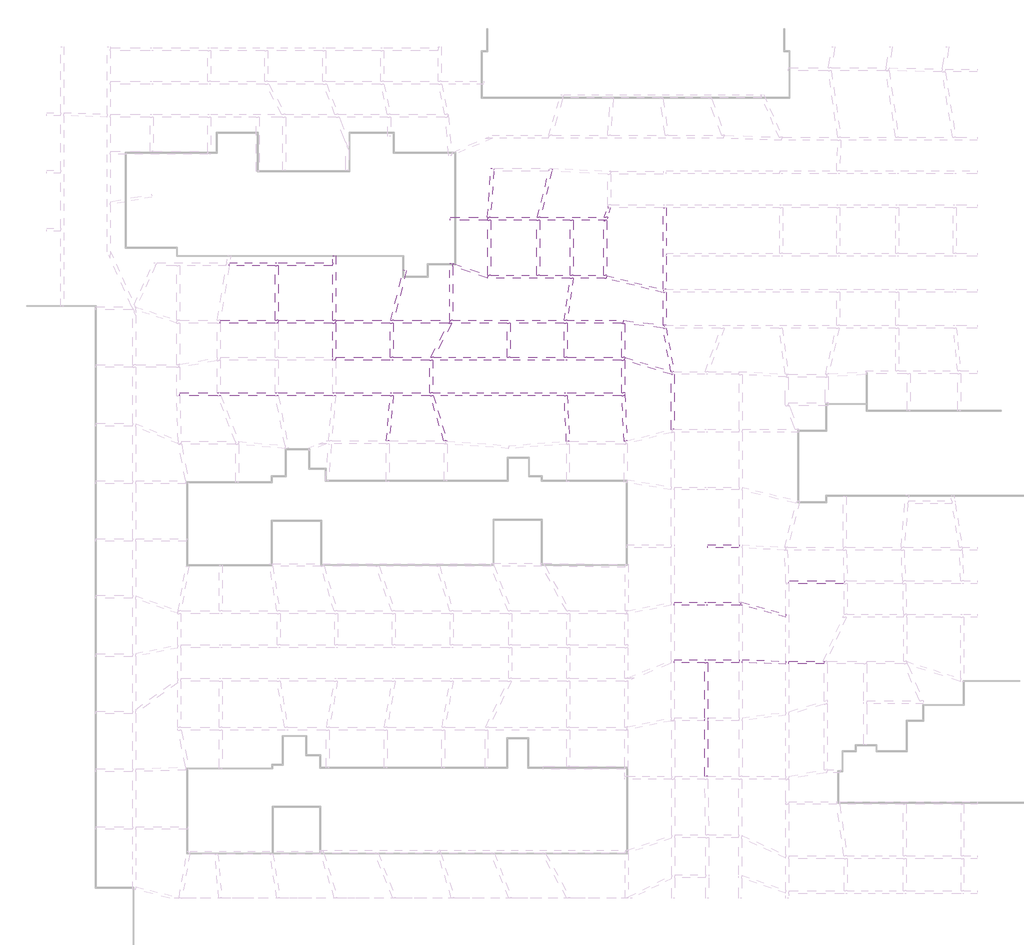
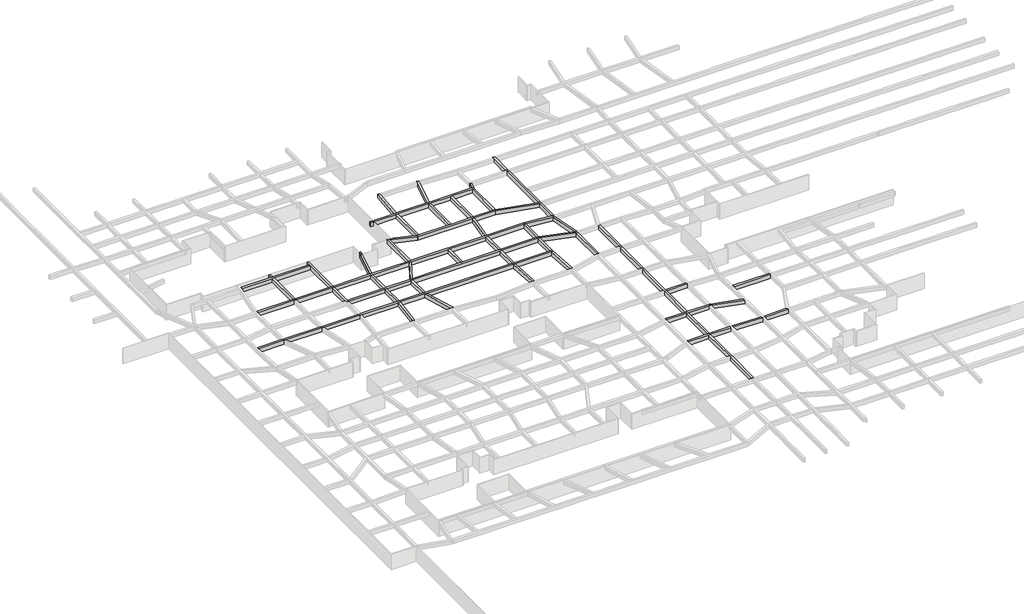
# One storey, part 16 of 45: 50 beams.
"""IFC4 building model written with IfcOpenShell, lengths in millimetres."""

from ifc_helpers import new_model, si_unit, frame, origin, place, context, project, spatial, polyline, outline, extrude, faceted_brep, element, save

model = new_model("IFC4")

# Units and contexts
model_context = context("Model", 3, world=origin())
ifc_project = project(units=[si_unit("LENGTHUNIT", "METRE", prefix="MILLI")], contexts=[model_context])

# Site, building, storey
site = spatial("IfcSite", under=ifc_project)
building = spatial("IfcBuilding", under=site)
storey = spatial("IfcBuildingStorey", under=building, Name="户型图", Elevation=0.0)

# Beams
placement = place(None, origin())
element("IfcBeam", 1, ObjectType="混凝土 - 矩形梁 : KL_beam", at=placement, inside=storey, context=model_context, shape_type="Brep", body=[
    faceted_brep([(-120998.6286131, -81886.7344834, 3300.0), (-120998.6286131, -81486.7344834, 3300.0), (-121398.6286131, -81486.7344834, 3300.0), (-128784.4586999, -81486.7344834, 3300.0), (-128818.6286131, -81486.7344834, 3300.0), (-128818.6286131, -81886.7344834, 3300.0), (-121398.6286131, -81886.7344834, 3300.0), (-120998.6286131, -81886.7344834, 2500.0), (-128818.6286131, -81886.7344834, 2500.0), (-121398.6286131, -81886.7344834, 2500.0), (-120998.6286131, -81486.7344834, 2500.0), (-128818.6286131, -81486.7344834, 2500.0), (-128784.4586999, -81486.7344834, 2500.0), (-121398.6286131, -81486.7344834, 2500.0)], [[[0, 1, 2, 3, 4, 5, 6]], [[7, 0, 6, 5, 8, 9]], [[10, 7, 9, 8, 11, 12, 13]], [[1, 10, 13, 12, 11, 4, 3, 2]], [[1, 0, 7, 10]], [[5, 4, 11, 8]]]),
])
element("IfcBeam", 2, ObjectType="混凝土 - 矩形梁 : KL_beam", at=placement, inside=storey, context=model_context, shape_type="Brep", body=[
    faceted_brep([(-113198.6286131, -81886.7344834, 3300.0), (-113198.6286131, -81486.7344834, 3300.0), (-113198.9292959, -81486.7344834, 3300.0), (-113598.9292959, -81486.7344834, 3300.0), (-120998.6286131, -81486.7344834, 3300.0), (-120998.6286131, -81886.7344834, 3300.0), (-113598.6286131, -81886.7344834, 3300.0), (-113198.6286131, -81886.7344834, 2500.0), (-120998.6286131, -81886.7344834, 2500.0), (-113598.6286131, -81886.7344834, 2500.0), (-113198.6286131, -81486.7344834, 2500.0), (-120998.6286131, -81486.7344834, 2500.0), (-113598.9292959, -81486.7344834, 2500.0), (-113198.9292959, -81486.7344834, 2500.0)], [[[0, 1, 2, 3, 4, 5, 6]], [[7, 0, 6, 5, 8, 9]], [[10, 7, 9, 8, 11, 12, 13]], [[1, 10, 13, 12, 11, 4, 3, 2]], [[5, 4, 11, 8]], [[1, 0, 7, 10]]]),
])
element("IfcBeam", 3, ObjectType="混凝土 - 矩形梁 : KL_beam", at=placement, inside=storey, context=model_context, shape_type="Brep", body=[
    faceted_brep([(-113598.6286131, -86886.7344834, 3300.0), (-113198.6286131, -86886.7344834, 3300.0), (-113198.6286131, -86486.7344834, 3300.0), (-113198.6286131, -81886.7344834, 3300.0), (-113598.6286131, -81886.7344834, 3300.0), (-113598.6286131, -86486.7344834, 3300.0), (-113598.6286131, -86886.7344834, 2500.0), (-113598.6286131, -81886.7344834, 2500.0), (-113598.6286131, -86486.7344834, 2500.0), (-113198.6286131, -86886.7344834, 2500.0), (-113198.6286131, -81886.7344834, 2500.0), (-113198.6286131, -86486.7344834, 2500.0)], [[[0, 1, 2, 3, 4, 5]], [[6, 0, 5, 4, 7, 8]], [[9, 6, 8, 7, 10, 11]], [[1, 9, 11, 10, 3, 2]], [[4, 3, 10, 7]], [[1, 0, 6, 9]]]),
])
element("IfcBeam", 4, ObjectType="混凝土 - 矩形梁 : KL_beam", at=placement, inside=storey, context=model_context, shape_type="SweptSolid", body=[
    extrude(outline(polyline([(-121398.6286131, -72759.2597696), (-120998.6286131, -72759.2597696), (-120998.6286131, -73686.7344834), (-121398.6286131, -73686.7344834), (-121398.6286131, -72759.2597696)])), frame((0.0, 0.0, 2500.0), z_axis=(0.0, 0.0, 1.0), x_axis=(1.0, 0.0, 0.0)), (0.0, 0.0, 1.0), 800.0),
    extrude(outline(polyline([(-120998.6286131, -81486.7344834), (-121398.6286131, -81486.7344834), (-121398.6286131, -74086.7344834), (-120998.6286131, -74086.7344834), (-120998.6286131, -81486.7344834)])), frame((0.0, 0.0, 2500.0), z_axis=(0.0, 0.0, 1.0), x_axis=(1.0, 0.0, 0.0)), (0.0, 0.0, 1.0), 800.0),
])
element("IfcBeam", 5, ObjectType="混凝土 - 矩形梁 : KL_beam", at=placement, inside=storey, context=model_context, shape_type="Brep", body=[
    faceted_brep([(-74128.0566076, -86886.7344834, 3300.0), (-74069.2006186, -86486.7344834, 3300.0), (-74098.3129002, -86486.7344834, 3300.0), (-74498.3129002, -86486.7344834, 3300.0), (-81898.3129002, -86486.7344834, 3300.0), (-82298.3129002, -86486.7344834, 3300.0), (-89598.3129002, -86486.7344834, 3300.0), (-89998.3129002, -86486.7344834, 3300.0), (-99914.2936835, -86486.7344834, 3300.0), (-100366.9162848, -86486.7344834, 3300.0), (-105392.6768411, -86486.7344834, 3300.0), (-105792.6768411, -86486.7344834, 3300.0), (-113198.6286131, -86486.7344834, 3300.0), (-113198.6286131, -86886.7344834, 3300.0), (-105792.6768411, -86886.7344834, 3300.0), (-105392.6768411, -86886.7344834, 3300.0), (-100446.5144021, -86886.7344834, 3300.0), (-100046.5144021, -86886.7344834, 3300.0), (-82298.3129002, -86886.7344834, 3300.0), (-81898.3129002, -86886.7344834, 3300.0), (-74498.3129002, -86886.7344834, 3300.0), (-74128.0566076, -86886.7344834, 2500.0), (-113198.6286131, -86886.7344834, 2500.0), (-105792.6768411, -86886.7344834, 2500.0), (-105392.6768411, -86886.7344834, 2500.0), (-100446.5144021, -86886.7344834, 2500.0), (-100046.5144021, -86886.7344834, 2500.0), (-82298.3129002, -86886.7344834, 2500.0), (-81898.3129002, -86886.7344834, 2500.0), (-74498.3129002, -86886.7344834, 2500.0), (-74069.2006186, -86486.7344834, 2500.0), (-113198.6286131, -86486.7344834, 2500.0), (-105792.6768411, -86486.7344834, 2500.0), (-105392.6768411, -86486.7344834, 2500.0), (-100366.9162848, -86486.7344834, 2500.0), (-99914.2936835, -86486.7344834, 2500.0), (-89998.3129002, -86486.7344834, 2500.0), (-89598.3129002, -86486.7344834, 2500.0), (-82298.3129002, -86486.7344834, 2500.0), (-81898.3129002, -86486.7344834, 2500.0), (-74498.3129002, -86486.7344834, 2500.0), (-74098.3129002, -86486.7344834, 2500.0)], [[[0, 1, 2, 3, 4, 5, 6, 7, 8, 9, 10, 11, 12, 13, 14, 15, 16, 17, 18, 19, 20]], [[21, 0, 20, 19, 18, 17, 16, 15, 14, 13, 22, 23, 24, 25, 26, 27, 28, 29]], [[30, 21, 29, 28, 27, 26, 25, 24, 23, 22, 31, 32, 33, 34, 35, 36, 37, 38, 39, 40, 41]], [[1, 30, 41, 40, 39, 38, 37, 36, 35, 34, 33, 32, 31, 12, 11, 10, 9, 8, 7, 6, 5, 4, 3, 2]], [[13, 12, 31, 22]], [[1, 0, 21, 30]]]),
])
element("IfcBeam", 6, ObjectType="混凝土 - 矩形梁 : KL_beam", at=placement, inside=storey, context=model_context, shape_type="Brep", body=[
    faceted_brep([(-74098.3129002, -91641.7669719, 3300.0), (-74098.3129002, -91436.9328993, 3300.0), (-74098.3129002, -91241.7669719, 3300.0), (-74498.3129002, -91241.7669719, 3300.0), (-81898.3129002, -91241.7669719, 3300.0), (-82298.3129002, -91241.7669719, 3300.0), (-100046.5144021, -91241.7669719, 3300.0), (-100446.5144021, -91241.7669719, 3300.0), (-105392.6768411, -91241.7669719, 3300.0), (-105792.6768411, -91241.7669719, 3300.0), (-113198.6286131, -91241.7669719, 3300.0), (-113598.6286131, -91241.7669719, 3300.0), (-120998.6286131, -91241.7669719, 3300.0), (-121398.6286131, -91241.7669719, 3300.0), (-128818.6286131, -91241.7669719, 3300.0), (-129218.6286131, -91241.7669719, 3300.0), (-134318.6286131, -91241.7669719, 3300.0), (-134318.6286131, -91641.7669719, 3300.0), (-134311.5225504, -91641.7669719, 3300.0), (-129156.0848049, -91641.7669719, 3300.0), (-128727.6268074, -91641.7669719, 3300.0), (-121363.4958903, -91641.7669719, 3300.0), (-120956.0092123, -91641.7669719, 3300.0), (-113616.8903133, -91641.7669719, 3300.0), (-113215.3623783, -91641.7669719, 3300.0), (-105810.9021134, -91641.7669719, 3300.0), (-105409.3741784, -91641.7669719, 3300.0), (-100395.5234862, -91641.7669719, 3300.0), (-99978.0743922, -91641.7669719, 3300.0), (-82288.8729227, -91641.7669719, 3300.0), (-81888.4052844, -91641.7669719, 3300.0), (-74488.8729227, -91641.7669719, 3300.0), (-74098.3129002, -91641.7669719, 2500.0), (-134318.6286131, -91641.7669719, 2500.0), (-134311.5225504, -91641.7669719, 2500.0), (-129156.0848049, -91641.7669719, 2500.0), (-128727.6268074, -91641.7669719, 2500.0), (-121363.4958903, -91641.7669719, 2500.0), (-120956.0092123, -91641.7669719, 2500.0), (-113616.8903133, -91641.7669719, 2500.0), (-113215.3623783, -91641.7669719, 2500.0), (-105810.9021134, -91641.7669719, 2500.0), (-105409.3741784, -91641.7669719, 2500.0), (-100395.5234862, -91641.7669719, 2500.0), (-99978.0743922, -91641.7669719, 2500.0), (-82288.8729227, -91641.7669719, 2500.0), (-81888.4052844, -91641.7669719, 2500.0), (-74488.8729227, -91641.7669719, 2500.0), (-74098.3129002, -91241.7669719, 2500.0), (-74098.3129002, -91436.9328993, 2500.0), (-134318.6286131, -91241.7669719, 2500.0), (-129218.6286131, -91241.7669719, 2500.0), (-128818.6286131, -91241.7669719, 2500.0), (-121398.6286131, -91241.7669719, 2500.0), (-120998.6286131, -91241.7669719, 2500.0), (-113598.6286131, -91241.7669719, 2500.0), (-113198.6286131, -91241.7669719, 2500.0), (-105792.6768411, -91241.7669719, 2500.0), (-105392.6768411, -91241.7669719, 2500.0), (-100446.5144021, -91241.7669719, 2500.0), (-100046.5144021, -91241.7669719, 2500.0), (-82298.3129002, -91241.7669719, 2500.0), (-81898.3129002, -91241.7669719, 2500.0), (-74498.3129002, -91241.7669719, 2500.0)], [[[0, 1, 2, 3, 4, 5, 6, 7, 8, 9, 10, 11, 12, 13, 14, 15, 16, 17, 18, 19, 20, 21, 22, 23, 24, 25, 26, 27, 28, 29, 30, 31]], [[32, 0, 31, 30, 29, 28, 27, 26, 25, 24, 23, 22, 21, 20, 19, 18, 17, 33, 34, 35, 36, 37, 38, 39, 40, 41, 42, 43, 44, 45, 46, 47]], [[48, 49, 32, 47, 46, 45, 44, 43, 42, 41, 40, 39, 38, 37, 36, 35, 34, 33, 50, 51, 52, 53, 54, 55, 56, 57, 58, 59, 60, 61, 62, 63]], [[2, 48, 63, 62, 61, 60, 59, 58, 57, 56, 55, 54, 53, 52, 51, 50, 16, 15, 14, 13, 12, 11, 10, 9, 8, 7, 6, 5, 4, 3]], [[17, 16, 50, 33]], [[2, 1, 0, 32, 49, 48]]]),
])
element("IfcBeam", 7, ObjectType="混凝土 - 矩形梁 : KL_beam", at=placement, inside=storey, context=model_context, shape_type="SweptSolid", body=[
    extrude(outline(polyline([(-105810.9021134, -91641.7669719), (-105409.3741784, -91641.7669719), (-105946.1060855, -97776.6407423), (-106347.6340205, -97776.6407423), (-105810.9021134, -91641.7669719)])), frame((0.0, 0.0, 2500.0), z_axis=(0.0, 0.0, 1.0), x_axis=(1.0, 0.0, 0.0)), (0.0, 0.0, 1.0), 800.0),
])
element("IfcBeam", 8, ObjectType="混凝土 - 矩形梁 : KL_beam", at=placement, inside=storey, context=model_context, shape_type="Brep", body=[
    faceted_brep([(-92598.5285941, -67552.5441851, 3300.0), (-92598.5285941, -67552.7981742, 3300.0), (-92598.5285941, -67952.5441851, 3300.0), (-92198.5285941, -67952.5441851, 3300.0), (-85971.6416274, -67952.5441851, 3300.0), (-85571.6416274, -67952.5441851, 3300.0), (-81471.6416274, -67952.5441851, 3300.0), (-81071.6416274, -67952.5441851, 3300.0), (-76547.2291492, -67952.5441851, 3300.0), (-76434.1522111, -67552.5441851, 3300.0), (-76849.828039, -67552.5441851, 3300.0), (-85515.5899744, -67552.5441851, 3300.0), (-85927.8354261, -67552.5441851, 3300.0), (-92270.5908787, -67552.5441851, 3300.0), (-92598.5285941, -67952.5441851, 2500.0), (-92198.5285941, -67952.5441851, 2500.0), (-85971.6416274, -67952.5441851, 2500.0), (-85571.6416274, -67952.5441851, 2500.0), (-81471.6416274, -67952.5441851, 2500.0), (-81071.6416274, -67952.5441851, 2500.0), (-76547.2291492, -67952.5441851, 2500.0), (-92598.5285941, -67552.7981742, 2500.0), (-92598.5285941, -67552.5441851, 2500.0), (-92270.5908787, -67552.5441851, 2500.0), (-85927.8354261, -67552.5441851, 2500.0), (-85515.5899744, -67552.5441851, 2500.0), (-76849.828039, -67552.5441851, 2500.0), (-76434.1522111, -67552.5441851, 2500.0)], [[[0, 1, 2, 3, 4, 5, 6, 7, 8, 9, 10, 11, 12, 13]], [[2, 14, 15, 16, 17, 18, 19, 20, 8, 7, 6, 5, 4, 3]], [[14, 21, 22, 23, 24, 25, 26, 27, 20, 19, 18, 17, 16, 15]], [[22, 0, 13, 12, 11, 10, 9, 27, 26, 25, 24, 23]], [[2, 1, 0, 22, 21, 14]], [[9, 8, 20, 27]]]),
])
element("IfcBeam", 9, ObjectType="混凝土 - 矩形梁 : KL_beam", at=placement, inside=storey, context=model_context, shape_type="Brep", body=[
    faceted_brep([(-92598.5285941, -75365.0521634, 3300.0), (-92598.5285941, -75765.0521634, 3300.0), (-81500.4649427, -75765.0521634, 3300.0), (-81096.8342659, -75765.0521634, 3300.0), (-76794.8911053, -75765.0521634, 3300.0), (-76570.1397921, -75765.0521634, 3300.0), (-76570.1397921, -75408.8435077, 3300.0), (-76570.1397921, -75365.0521634, 3300.0), (-76970.1397921, -75365.0521634, 3300.0), (-81071.6416274, -75365.0521634, 3300.0), (-81471.6416274, -75365.0521634, 3300.0), (-85571.6416274, -75365.0521634, 3300.0), (-85971.6416274, -75365.0521634, 3300.0), (-92198.5285941, -75365.0521634, 3300.0), (-92598.5285941, -75765.0521634, 2500.0), (-81500.4649427, -75765.0521634, 2500.0), (-81096.8342659, -75765.0521634, 2500.0), (-76794.8911053, -75765.0521634, 2500.0), (-76570.1397921, -75765.0521634, 2500.0), (-92598.5285941, -75365.0521634, 2500.0), (-92198.5285941, -75365.0521634, 2500.0), (-85971.6416274, -75365.0521634, 2500.0), (-85571.6416274, -75365.0521634, 2500.0), (-81471.6416274, -75365.0521634, 2500.0), (-81071.6416274, -75365.0521634, 2500.0), (-76970.1397921, -75365.0521634, 2500.0), (-76570.1397921, -75365.0521634, 2500.0), (-76570.1397921, -75408.8435077, 2500.0)], [[[0, 1, 2, 3, 4, 5, 6, 7, 8, 9, 10, 11, 12, 13]], [[1, 14, 15, 16, 17, 18, 5, 4, 3, 2]], [[14, 19, 20, 21, 22, 23, 24, 25, 26, 27, 18, 17, 16, 15]], [[19, 0, 13, 12, 11, 10, 9, 8, 7, 26, 25, 24, 23, 22, 21, 20]], [[1, 0, 19, 14]], [[7, 6, 5, 18, 27, 26]]]),
])
element("IfcBeam", 10, ObjectType="混凝土 - 矩形梁 : KL_beam", at=placement, inside=storey, context=model_context, shape_type="Brep", body=[
    faceted_brep([(-74310.2286213, -81886.7344834, 3300.0), (-74287.028605, -81486.7344834, 3300.0), (-81869.489585, -81486.7344834, 3300.0), (-82273.1202618, -81486.7344834, 3300.0), (-97398.6286131, -81486.7344834, 3300.0), (-97798.6286131, -81486.7344834, 3300.0), (-97798.6286131, -81886.7344834, 3300.0), (-97478.3770718, -81886.7344834, 3300.0), (-89998.3129002, -81886.7344834, 3300.0), (-89598.3129002, -81886.7344834, 3300.0), (-82298.3129002, -81886.7344834, 3300.0), (-81898.3129002, -81886.7344834, 3300.0), (-74498.3129002, -81886.7344834, 3300.0), (-74310.2286213, -81886.7344834, 2500.0), (-97798.6286131, -81886.7344834, 2500.0), (-97478.3770718, -81886.7344834, 2500.0), (-89998.3129002, -81886.7344834, 2500.0), (-89598.3129002, -81886.7344834, 2500.0), (-82298.3129002, -81886.7344834, 2500.0), (-81898.3129002, -81886.7344834, 2500.0), (-74498.3129002, -81886.7344834, 2500.0), (-74287.028605, -81486.7344834, 2500.0), (-97798.6286131, -81486.7344834, 2500.0), (-97398.6286131, -81486.7344834, 2500.0), (-82273.1202618, -81486.7344834, 2500.0), (-81869.489585, -81486.7344834, 2500.0)], [[[0, 1, 2, 3, 4, 5, 6, 7, 8, 9, 10, 11, 12]], [[13, 0, 12, 11, 10, 9, 8, 7, 6, 14, 15, 16, 17, 18, 19, 20]], [[21, 13, 20, 19, 18, 17, 16, 15, 14, 22, 23, 24, 25]], [[1, 21, 25, 24, 23, 22, 5, 4, 3, 2]], [[1, 0, 13, 21]], [[6, 5, 22, 14]]]),
])
element("IfcBeam", 11, ObjectType="混凝土 - 矩形梁 : KL_beam", at=placement, inside=storey, context=model_context, shape_type="SweptSolid", body=[
    extrude(outline(polyline([(-85971.6416274, -67952.5441851), (-85571.6416274, -67952.5441851), (-85571.6416274, -75365.0521634), (-85971.6416274, -75365.0521634), (-85971.6416274, -67952.5441851)])), frame((0.0, 0.0, 2500.0), z_axis=(0.0, 0.0, 1.0), x_axis=(1.0, 0.0, 0.0)), (0.0, 0.0, 1.0), 800.0),
])
element("IfcBeam", 12, ObjectType="混凝土 - 矩形梁 : KL_beam", at=placement, inside=storey, context=model_context, shape_type="SweptSolid", body=[
    extrude(outline(polyline([(-81471.6416274, -67952.5441851), (-81071.6416274, -67952.5441851), (-81071.6416274, -75365.0521634), (-81471.6416274, -75365.0521634), (-81471.6416274, -67952.5441851)])), frame((0.0, 0.0, 2500.0), z_axis=(0.0, 0.0, 1.0), x_axis=(1.0, 0.0, 0.0)), (0.0, 0.0, 1.0), 800.0),
])
element("IfcBeam", 13, ObjectType="混凝土 - 矩形梁 : KL_beam", at=placement, inside=storey, context=model_context, shape_type="Brep", body=[
    faceted_brep([(-92198.5285941, -67952.5441851, 3300.0), (-92598.5285941, -67952.5441851, 3300.0), (-92598.5285941, -67952.7981742, 3300.0), (-92598.5285941, -75353.8354852, 3300.0), (-92598.5285941, -75365.0521634, 3300.0), (-92198.5285941, -75365.0521634, 3300.0), (-92598.5285941, -67952.5441851, 2500.0), (-92598.5285941, -67952.7981742, 2500.0), (-92598.5285941, -75353.8354852, 2500.0), (-92598.5285941, -75365.0521634, 2500.0), (-92198.5285941, -67952.5441851, 2500.0), (-92198.5285941, -75365.0521634, 2500.0)], [[[0, 1, 2, 3, 4, 5]], [[1, 6, 7, 8, 9, 4, 3, 2]], [[6, 10, 11, 9, 8, 7]], [[10, 0, 5, 11]], [[1, 0, 10, 6]], [[5, 4, 9, 11]]]),
])
element("IfcBeam", 14, ObjectType="混凝土 - 矩形梁 : KL_beam", at=placement, inside=storey, context=model_context, shape_type="Brep", body=[
    faceted_brep([(-68721.961123, -82134.4617231, 3300.0), (-68900.6999587, -82113.6580198, 3300.0), (-74287.028605, -81486.7344834, 3300.0), (-74310.2286213, -81886.7344834, 3300.0), (-74098.3129002, -81911.3996982, 3300.0), (-68904.9700465, -82515.8613049, 3300.0), (-68745.1611393, -82534.4617231, 3300.0), (-74310.2286213, -81886.7344834, 2500.0), (-74098.3129002, -81911.3996982, 2500.0), (-68904.9700465, -82515.8613049, 2500.0), (-68745.1611393, -82534.4617231, 2500.0), (-74287.028605, -81486.7344834, 2500.0), (-68900.6999587, -82113.6580198, 2500.0), (-68721.961123, -82134.4617231, 2500.0)], [[[0, 1, 2, 3, 4, 5, 6]], [[6, 5, 4, 3, 7, 8, 9, 10]], [[10, 9, 8, 7, 11, 12, 13]], [[2, 1, 0, 13, 12, 11]], [[2, 11, 7, 3]], [[0, 6, 10, 13]]]),
])
element("IfcBeam", 15, ObjectType="混凝土 - 矩形梁 : KL_beam", at=placement, inside=storey, context=model_context, shape_type="Brep", body=[
    faceted_brep([(-67740.4118212, -88390.3844516, 3300.0), (-67876.3425814, -88349.4975464, 3300.0), (-74069.2006186, -86486.7344834, 3300.0), (-74128.0566076, -86886.7344834, 3300.0), (-74098.3129002, -86895.681157, 3300.0), (-67830.7823984, -88780.9051109, 3300.0), (-67799.2678102, -88790.3844516, 3300.0), (-74128.0566076, -86886.7344834, 2500.0), (-74098.3129002, -86895.681157, 2500.0), (-67830.7823984, -88780.9051109, 2500.0), (-67799.2678102, -88790.3844516, 2500.0), (-74069.2006186, -86486.7344834, 2500.0), (-67876.3425814, -88349.4975464, 2500.0), (-67740.4118212, -88390.3844516, 2500.0)], [[[0, 1, 2, 3, 4, 5, 6]], [[6, 5, 4, 3, 7, 8, 9, 10]], [[10, 9, 8, 7, 11, 12, 13]], [[2, 1, 0, 13, 12, 11]], [[2, 11, 7, 3]], [[0, 6, 10, 13]]]),
])
element("IfcBeam", 16, ObjectType="混凝土 - 矩形梁 : KL_beam", at=placement, inside=storey, context=model_context, shape_type="SweptSolid", body=[
    extrude(outline(polyline([(-74310.2286213, -81886.7344834), (-74098.3129002, -81911.3996982), (-74098.3129002, -86486.7344834), (-74498.3129002, -86486.7344834), (-74498.3129002, -81886.7344834), (-74310.2286213, -81886.7344834)])), frame((0.0, 0.0, 2500.0), z_axis=(0.0, 0.0, 1.0), x_axis=(1.0, 0.0, 0.0)), (0.0, 0.0, 1.0), 800.0),
])
element("IfcBeam", 17, ObjectType="混凝土 - 矩形梁 : KL_beam", at=placement, inside=storey, context=model_context, shape_type="SweptSolid", body=[
    extrude(outline(polyline([(-74098.3129002, -91241.7669719), (-74498.3129002, -91241.7669719), (-74498.3129002, -86886.7344834), (-74128.0566076, -86886.7344834), (-74098.3129002, -86895.681157), (-74098.3129002, -91241.7669719)])), frame((0.0, 0.0, 2500.0), z_axis=(0.0, 0.0, 1.0), x_axis=(1.0, 0.0, 0.0)), (0.0, 0.0, 1.0), 800.0),
])
element("IfcBeam", 18, ObjectType="混凝土 - 矩形梁 : KL_beam", at=placement, inside=storey, context=model_context, shape_type="SweptSolid", body=[
    extrude(outline(polyline([(-74488.8729227, -91641.7669719), (-74098.3129002, -91641.7669719), (-74098.3129002, -91436.9328993), (-73792.8353015, -97752.5007811), (-74005.7852131, -97806.5978244), (-74190.6863209, -97806.5978244), (-74488.8729227, -91641.7669719)])), frame((0.0, 0.0, 2500.0), z_axis=(0.0, 0.0, 1.0), x_axis=(1.0, 0.0, 0.0)), (0.0, 0.0, 1.0), 800.0),
])
element("IfcBeam", 19, ObjectType="混凝土 - 矩形梁 : KL_beam", at=placement, inside=storey, context=model_context, shape_type="SweptSolid", body=[
    extrude(outline(polyline([(-81590.2186825, -97806.5978244), (-81990.6863209, -97806.5978244), (-82288.8729227, -91641.7669719), (-81888.4052844, -91641.7669719), (-81590.2186825, -97806.5978244)])), frame((0.0, 0.0, 2500.0), z_axis=(0.0, 0.0, 1.0), x_axis=(1.0, 0.0, 0.0)), (0.0, 0.0, 1.0), 800.0),
])
element("IfcBeam", 20, ObjectType="混凝土 - 矩形梁 : KL_beam", at=placement, inside=storey, context=model_context, shape_type="SweptSolid", body=[
    extrude(outline(polyline([(-81898.3129002, -91241.7669719), (-82298.3129002, -91241.7669719), (-82298.3129002, -86886.7344834), (-81898.3129002, -86886.7344834), (-81898.3129002, -91241.7669719)])), frame((0.0, 0.0, 2500.0), z_axis=(0.0, 0.0, 1.0), x_axis=(1.0, 0.0, 0.0)), (0.0, 0.0, 1.0), 800.0),
    extrude(outline(polyline([(-82298.3129002, -81886.7344834), (-81898.3129002, -81886.7344834), (-81898.3129002, -86486.7344834), (-82298.3129002, -86486.7344834), (-82298.3129002, -81886.7344834)])), frame((0.0, 0.0, 2500.0), z_axis=(0.0, 0.0, 1.0), x_axis=(1.0, 0.0, 0.0)), (0.0, 0.0, 1.0), 800.0),
])
element("IfcBeam", 21, ObjectType="混凝土 - 矩形梁 : KL_beam", at=placement, inside=storey, context=model_context, shape_type="SweptSolid", body=[
    extrude(outline(polyline([(-81500.4649427, -75765.0521634), (-81096.8342659, -75765.0521634), (-81869.489585, -81486.7344834), (-82273.1202618, -81486.7344834), (-81500.4649427, -75765.0521634)])), frame((0.0, 0.0, 2500.0), z_axis=(0.0, 0.0, 1.0), x_axis=(1.0, 0.0, 0.0)), (0.0, 0.0, 1.0), 800.0),
])
element("IfcBeam", 22, ObjectType="混凝土 - 矩形梁 : KL_beam", at=placement, inside=storey, context=model_context, shape_type="SweptSolid", body=[
    extrude(outline(polyline([(-89598.3129002, -86486.7344834), (-89998.3129002, -86486.7344834), (-89998.3129002, -81886.7344834), (-89598.3129002, -81886.7344834), (-89598.3129002, -86486.7344834)])), frame((0.0, 0.0, 2500.0), z_axis=(0.0, 0.0, 1.0), x_axis=(1.0, 0.0, 0.0)), (0.0, 0.0, 1.0), 800.0),
])
element("IfcBeam", 23, ObjectType="混凝土 - 矩形梁 : KL_beam", at=placement, inside=storey, context=model_context, shape_type="SweptSolid", body=[
    extrude(outline(polyline([(-68904.9700465, -82515.8613049), (-68745.1611393, -82534.4617231), (-68495.5196461, -82534.4617231), (-67462.9624722, -88390.3844516), (-67740.4118212, -88390.3844516), (-67876.3425814, -88349.4975464), (-68904.9700465, -82515.8613049)])), frame((0.0, 0.0, 2500.0), z_axis=(0.0, 0.0, 1.0), x_axis=(1.0, 0.0, 0.0)), (0.0, 0.0, 1.0), 800.0),
])
element("IfcBeam", 24, ObjectType="混凝土 - 矩形梁 : KL_beam", at=placement, inside=storey, context=model_context, shape_type="Brep", body=[
    faceted_brep([(-67725.9320986, -96211.286122, 3300.0), (-67430.7823984, -96211.286122, 3300.0), (-67430.7823984, -88790.3844516, 3300.0), (-67798.6023246, -88790.3844516, 3300.0), (-67799.2678102, -88790.3844516, 3300.0), (-67830.7823984, -88780.9051109, 3300.0), (-67830.7823984, -96237.9219218, 3300.0), (-67830.7823984, -88780.9051109, 2500.0), (-67830.7823984, -96237.9219218, 2500.0), (-67430.7823984, -96211.286122, 2500.0), (-67725.9320986, -96211.286122, 2500.0), (-67799.2678102, -88790.3844516, 2500.0), (-67798.6023246, -88790.3844516, 2500.0), (-67430.7823984, -88790.3844516, 2500.0)], [[[0, 1, 2, 3, 4, 5, 6]], [[5, 7, 8, 6]], [[9, 10, 8, 7, 11, 12, 13]], [[1, 9, 13, 2]], [[1, 0, 10, 9]], [[2, 13, 12, 11, 4, 3]], [[5, 4, 11, 7]], [[0, 6, 8, 10]]]),
])
element("IfcBeam", 25, ObjectType="混凝土 - 矩形梁 : KL_beam", at=placement, inside=storey, context=model_context, shape_type="Brep", body=[
    faceted_brep([(-58457.1128979, -119970.4077047, 3300.0), (-58404.4518989, -119570.4077047, 3300.0), (-58630.7823984, -119570.4077047, 3300.0), (-62877.6696197, -119570.4077047, 3300.0), (-63277.6696197, -119570.4077047, 3300.0), (-67430.7823984, -119570.4077047, 3300.0), (-67430.7823984, -119970.4077047, 3300.0), (-63277.6696197, -119970.4077047, 3300.0), (-62877.6696197, -119970.4077047, 3300.0), (-58630.7823984, -119970.4077047, 3300.0), (-58457.1128979, -119970.4077047, 2500.0), (-67430.7823984, -119970.4077047, 2500.0), (-63277.6696197, -119970.4077047, 2500.0), (-62877.6696197, -119970.4077047, 2500.0), (-58630.7823984, -119970.4077047, 2500.0), (-58404.4518989, -119570.4077047, 2500.0), (-67430.7823984, -119570.4077047, 2500.0), (-63277.6696197, -119570.4077047, 2500.0), (-62877.6696197, -119570.4077047, 2500.0), (-58630.7823984, -119570.4077047, 2500.0)], [[[0, 1, 2, 3, 4, 5, 6, 7, 8, 9]], [[10, 0, 9, 8, 7, 6, 11, 12, 13, 14]], [[15, 10, 14, 13, 12, 11, 16, 17, 18, 19]], [[1, 15, 19, 18, 17, 16, 5, 4, 3, 2]], [[6, 5, 16, 11]], [[1, 0, 10, 15]]]),
])
element("IfcBeam", 26, ObjectType="混凝土 - 矩形梁 : KL_beam", at=placement, inside=storey, context=model_context, shape_type="Brep", body=[
    faceted_brep([(-67430.7823984, -127365.3480623, 3300.0), (-67430.7823984, -127765.3480623, 3300.0), (-63277.6696197, -127765.3480623, 3300.0), (-62877.6696197, -127765.3480623, 3300.0), (-58630.7823984, -127765.3480623, 3300.0), (-58630.7823984, -127365.3480623, 3300.0), (-62877.6696197, -127365.3480623, 3300.0), (-63277.6696197, -127365.3480623, 3300.0), (-67430.7823984, -127765.3480623, 2500.0), (-63277.6696197, -127765.3480623, 2500.0), (-62877.6696197, -127765.3480623, 2500.0), (-58630.7823984, -127765.3480623, 2500.0), (-67430.7823984, -127365.3480623, 2500.0), (-63277.6696197, -127365.3480623, 2500.0), (-62877.6696197, -127365.3480623, 2500.0), (-58630.7823984, -127365.3480623, 2500.0)], [[[0, 1, 2, 3, 4, 5, 6, 7]], [[1, 8, 9, 10, 11, 4, 3, 2]], [[8, 12, 13, 14, 15, 11, 10, 9]], [[12, 0, 7, 6, 5, 15, 14, 13]], [[1, 0, 12, 8]], [[5, 4, 11, 15]]]),
])
element("IfcBeam", 27, ObjectType="混凝土 - 矩形梁 : KL_beam", at=placement, inside=storey, context=model_context, shape_type="SweptSolid", body=[
    extrude(outline(polyline([(-58230.7823984, -127768.9840855), (-58230.7823984, -127368.7402678), (-52297.3620817, -127575.9398709), (-52297.3620817, -127976.1836887), (-58230.7823984, -127768.9840855)])), frame((0.0, 0.0, 2500.0), z_axis=(0.0, 0.0, 1.0), x_axis=(1.0, 0.0, 0.0)), (0.0, 0.0, 1.0), 800.0),
])
element("IfcBeam", 28, ObjectType="混凝土 - 矩形梁 : KL_beam", at=placement, inside=storey, context=model_context, shape_type="Brep", body=[
    faceted_brep([(-58404.4518989, -119570.4077047, 3300.0), (-58457.1128979, -119970.4077047, 3300.0), (-58230.7823984, -120031.0527792, 3300.0), (-52297.3620817, -121620.9079614, 3300.0), (-52297.3620817, -121206.7974893, 3300.0), (-58230.7823984, -119616.9423071, 3300.0), (-58457.1128979, -119970.4077047, 2500.0), (-58230.7823984, -120031.0527792, 2500.0), (-52297.3620817, -121620.9079614, 2500.0), (-58404.4518989, -119570.4077047, 2500.0), (-58230.7823984, -119616.9423071, 2500.0), (-52297.3620817, -121206.7974893, 2500.0)], [[[0, 1, 2, 3, 4, 5]], [[1, 6, 7, 8, 3, 2]], [[6, 9, 10, 11, 8, 7]], [[9, 0, 5, 4, 11, 10]], [[0, 9, 6, 1]], [[4, 3, 8, 11]]]),
])
element("IfcBeam", 29, ObjectType="混凝土 - 矩形梁 : KL_beam", at=placement, inside=storey, context=model_context, shape_type="Brep", body=[
    faceted_brep([(-47087.6738698, -127942.8806028, 3300.0), (-47087.6738698, -127542.8806028, 3300.0), (-47222.4961059, -127542.8806028, 3300.0), (-51897.3620817, -127542.8806028, 3300.0), (-51897.3620817, -127942.8806028, 3300.0), (-47087.6738698, -127542.8806028, 2500.0), (-47222.4961059, -127542.8806028, 2500.0), (-51897.3620817, -127542.8806028, 2500.0), (-47087.6738698, -127942.8806028, 2500.0), (-51897.3620817, -127942.8806028, 2500.0)], [[[0, 1, 2, 3, 4]], [[1, 5, 6, 7, 3, 2]], [[5, 8, 9, 7, 6]], [[8, 0, 4, 9]], [[1, 0, 8, 5]], [[3, 7, 9, 4]]]),
])
element("IfcBeam", 30, ObjectType="混凝土 - 矩形梁 : KL_beam", at=placement, inside=storey, context=model_context, shape_type="Brep", body=[
    faceted_brep([(-51907.4445387, -116668.4603553, 3300.0), (-51886.481427, -117068.4603553, 3300.0), (-44392.4702803, -117068.4603553, 3300.0), (-44385.6244664, -117068.4603553, 3300.0), (-44399.5927742, -116668.4603553, 3300.0), (-51886.481427, -117068.4603553, 2500.0), (-44392.4702803, -117068.4603553, 2500.0), (-44385.6244664, -117068.4603553, 2500.0), (-51907.4445387, -116668.4603553, 2500.0), (-44399.5927742, -116668.4603553, 2500.0)], [[[0, 1, 2, 3, 4]], [[1, 5, 6, 7, 3, 2]], [[5, 8, 9, 7, 6]], [[8, 0, 4, 9]], [[1, 0, 8, 5]], [[4, 3, 7, 9]]]),
])
element("IfcBeam", 31, ObjectType="混凝土 - 矩形梁 : KL_beam", at=placement, inside=storey, context=model_context, shape_type="SweptSolid", body=[
    extrude(outline(polyline([(-58630.7823984, -111828.4346923), (-58630.7823984, -112228.4346923), (-62877.6696197, -112228.4346923), (-62877.6696197, -111828.4346923), (-58630.7823984, -111828.4346923)])), frame((0.0, 0.0, 2500.0), z_axis=(0.0, 0.0, 1.0), x_axis=(1.0, 0.0, 0.0)), (0.0, 0.0, 1.0), 800.0),
])
element("IfcBeam", 32, ObjectType="混凝土 - 矩形梁 : KL_beam", at=placement, inside=storey, context=model_context, shape_type="SweptSolid", body=[
    extrude(outline(polyline([(-105392.6768411, -91241.7669719), (-105792.6768411, -91241.7669719), (-105792.6768411, -86886.7344834), (-105392.6768411, -86886.7344834), (-105392.6768411, -91241.7669719)])), frame((0.0, 0.0, 2500.0), z_axis=(0.0, 0.0, 1.0), x_axis=(1.0, 0.0, 0.0)), (0.0, 0.0, 1.0), 800.0),
    extrude(outline(polyline([(-105392.6768411, -86486.7344834), (-105792.6768411, -86486.7344834), (-105792.6768411, -81886.7344834), (-105392.6768411, -81886.7344834), (-105392.6768411, -86486.7344834)])), frame((0.0, 0.0, 2500.0), z_axis=(0.0, 0.0, 1.0), x_axis=(1.0, 0.0, 0.0)), (0.0, 0.0, 1.0), 800.0),
])
element("IfcBeam", 33, ObjectType="混凝土 - 矩形梁 : KL_beam", at=placement, inside=storey, context=model_context, shape_type="SweptSolid", body=[
    extrude(outline(polyline([(-104045.0172739, -74652.7141451), (-103656.8989834, -74749.4829033), (-105336.6844645, -81486.7344834), (-105748.9299162, -81486.7344834), (-104045.0172739, -74652.7141451)])), frame((0.0, 0.0, 2500.0), z_axis=(0.0, 0.0, 1.0), x_axis=(1.0, 0.0, 0.0)), (0.0, 0.0, 1.0), 800.0),
])
element("IfcBeam", 34, ObjectType="混凝土 - 矩形梁 : KL_beam", at=placement, inside=storey, context=model_context, shape_type="Brep", body=[
    faceted_brep([(-113198.6286131, -81486.7344834, 3300.0), (-113198.6286131, -81886.7344834, 3300.0), (-105792.6768411, -81886.7344834, 3300.0), (-105392.6768411, -81886.7344834, 3300.0), (-97930.999673, -81886.7344834, 3300.0), (-97798.6286131, -81886.7344834, 3300.0), (-97798.6286131, -81486.7344834, 3300.0), (-105336.6844645, -81486.7344834, 3300.0), (-105748.9299162, -81486.7344834, 3300.0), (-113198.6286131, -81486.7344834, 2500.0), (-97798.6286131, -81486.7344834, 2500.0), (-105336.6844645, -81486.7344834, 2500.0), (-105748.9299162, -81486.7344834, 2500.0), (-113198.6286131, -81886.7344834, 2500.0), (-97798.6286131, -81886.7344834, 2500.0), (-97930.999673, -81886.7344834, 2500.0), (-105392.6768411, -81886.7344834, 2500.0), (-105792.6768411, -81886.7344834, 2500.0)], [[[0, 1, 2, 3, 4, 5, 6, 7, 8]], [[9, 0, 8, 7, 6, 10, 11, 12]], [[13, 9, 12, 11, 10, 14, 15, 16, 17]], [[1, 13, 17, 16, 15, 14, 5, 4, 3, 2]], [[1, 0, 9, 13]], [[6, 5, 14, 10]]]),
])
element("IfcBeam", 35, ObjectType="混凝土 - 矩形梁 : KL_beam", at=placement, inside=storey, context=model_context, shape_type="Brep", body=[
    faceted_brep([(-127549.0600654, -73686.7344834, 3300.0), (-127612.4138415, -74086.7344834, 3300.0), (-121398.6286131, -74086.7344834, 3300.0), (-120998.6286131, -74086.7344834, 3300.0), (-113598.9292959, -74086.7344834, 3300.0), (-113598.9292959, -73686.7344834, 3300.0), (-120998.6286131, -73686.7344834, 3300.0), (-121398.6286131, -73686.7344834, 3300.0), (-127549.0600654, -73686.7344834, 2500.0), (-113598.9292959, -73686.7344834, 2500.0), (-120998.6286131, -73686.7344834, 2500.0), (-121398.6286131, -73686.7344834, 2500.0), (-127612.4138415, -74086.7344834, 2500.0), (-113598.9292959, -74086.7344834, 2500.0), (-120998.6286131, -74086.7344834, 2500.0), (-121398.6286131, -74086.7344834, 2500.0)], [[[0, 1, 2, 3, 4, 5, 6, 7]], [[8, 0, 7, 6, 5, 9, 10, 11]], [[12, 8, 11, 10, 9, 13, 14, 15]], [[1, 12, 15, 14, 13, 4, 3, 2]], [[1, 0, 8, 12]], [[5, 4, 13, 9]]]),
])
element("IfcBeam", 36, ObjectType="混凝土 - 矩形梁 : KL_beam", at=placement, inside=storey, context=model_context, shape_type="Brep", body=[
    faceted_brep([(-113198.9292959, -72759.2597696, 3300.0), (-113198.9292959, -72759.2597696, 2500.0), (-113598.9292959, -72759.2597696, 2500.0), (-113598.9292959, -72759.2597696, 3300.0), (-113598.9292959, -73686.7344834, 3300.0), (-113598.9292959, -74086.7344834, 3300.0), (-113598.9292959, -81486.7344834, 3300.0), (-113198.9292959, -81486.7344834, 3300.0), (-113598.9292959, -73686.7344834, 2500.0), (-113598.9292959, -74086.7344834, 2500.0), (-113598.9292959, -81486.7344834, 2500.0), (-113198.9292959, -81486.7344834, 2500.0)], [[[0, 1, 2, 3]], [[0, 3, 4, 5, 6, 7]], [[3, 2, 8, 9, 10, 6, 5, 4]], [[2, 1, 11, 10, 9, 8]], [[1, 0, 7, 11]], [[7, 6, 10, 11]]]),
])
element("IfcBeam", 37, ObjectType="混凝土 - 矩形梁 : KL_beam", at=placement, inside=storey, context=model_context, shape_type="Brep", body=[
    faceted_brep([(-97398.6286131, -73742.8929993, 3300.0), (-97798.6286131, -73742.8929993, 3300.0), (-97798.6286131, -81486.7344834, 3300.0), (-97398.6286131, -81486.7344834, 3300.0), (-97398.6286131, -74164.8183773, 3300.0), (-97398.6286131, -73742.8929993, 2500.0), (-97398.6286131, -81486.7344834, 2500.0), (-97398.6286131, -74164.8183773, 2500.0), (-97798.6286131, -73742.8929993, 2500.0), (-97798.6286131, -81486.7344834, 2500.0)], [[[0, 1, 2, 3, 4]], [[5, 0, 4, 3, 6, 7]], [[8, 5, 7, 6, 9]], [[1, 8, 9, 2]], [[3, 2, 9, 6]], [[1, 0, 5, 8]]]),
])
element("IfcBeam", 38, ObjectType="混凝土 - 矩形梁 : KL_beam", at=placement, inside=storey, context=model_context, shape_type="Brep", body=[
    faceted_brep([(-97398.6286131, -74164.8183773, 3300.0), (-92630.4371389, -75765.0521634, 3300.0), (-92598.5285941, -75765.0521634, 3300.0), (-92598.5285941, -75365.0521634, 3300.0), (-92598.5285941, -75353.8354852, 3300.0), (-97398.6286131, -73742.8929993, 3300.0), (-92630.4371389, -75765.0521634, 2500.0), (-97398.6286131, -74164.8183773, 2500.0), (-97398.6286131, -73742.8929993, 2500.0), (-92598.5285941, -75353.8354852, 2500.0), (-92598.5285941, -75365.0521634, 2500.0), (-92598.5285941, -75765.0521634, 2500.0)], [[[0, 1, 2, 3, 4, 5]], [[6, 1, 0, 7]], [[6, 7, 8, 9, 10, 11]], [[8, 5, 4, 9]], [[1, 6, 11, 2]], [[0, 5, 8, 7]], [[4, 3, 2, 11, 10, 9]]]),
])
element("IfcBeam", 39, ObjectType="混凝土 - 矩形梁 : KL_beam", at=placement, inside=storey, context=model_context, shape_type="Brep", body=[
    faceted_brep([(-97698.5285941, -67952.7981742, 3300.0), (-97698.5285941, -67552.7981742, 3300.0), (-97698.5285941, -67552.7981742, 2500.0), (-97698.5285941, -67952.7981742, 2500.0), (-92598.5285941, -67952.7981742, 3300.0), (-92598.5285941, -67952.5441851, 3300.0), (-92598.5285941, -67552.7981742, 3300.0), (-92671.5853986, -67552.7981742, 3300.0), (-92598.5285941, -67552.7981742, 2500.0), (-92671.5853986, -67552.7981742, 2500.0), (-92598.5285941, -67952.5441851, 2500.0), (-92598.5285941, -67952.7981742, 2500.0)], [[[0, 1, 2, 3]], [[1, 0, 4, 5, 6, 7]], [[2, 1, 7, 6, 8, 9]], [[3, 2, 9, 8, 10, 11]], [[0, 3, 11, 4]], [[4, 11, 10, 8, 6, 5]]]),
])
element("IfcBeam", 40, ObjectType="混凝土 - 矩形梁 : KL_beam", at=placement, inside=storey, context=model_context, shape_type="Brep", body=[
    faceted_brep([(-92598.5285941, -67552.5441851, 3300.0), (-92270.5908787, -67552.5441851, 3300.0), (-91832.5179464, -61287.8093836, 3300.0), (-91804.5472216, -60887.8093836, 3300.0), (-92205.5239808, -60887.8093836, 3300.0), (-92671.5853986, -67552.7981742, 3300.0), (-92598.5285941, -67552.7981742, 3300.0), (-92205.5239808, -60887.8093836, 2500.0), (-92671.5853986, -67552.7981742, 2500.0), (-92270.5908787, -67552.5441851, 2500.0), (-92598.5285941, -67552.5441851, 2500.0), (-92598.5285941, -67552.7981742, 2500.0), (-91804.5472216, -60887.8093836, 2500.0), (-91832.5179464, -61287.8093836, 2500.0)], [[[0, 1, 2, 3, 4, 5, 6]], [[4, 7, 8, 5]], [[9, 10, 11, 8, 7, 12, 13]], [[1, 9, 13, 12, 3, 2]], [[0, 10, 9, 1]], [[6, 5, 8, 11]], [[10, 0, 6, 11]], [[4, 3, 12, 7]]]),
])
element("IfcBeam", 41, ObjectType="混凝土 - 矩形梁 : KL_beam", at=placement, inside=storey, context=model_context, shape_type="Brep", body=[
    faceted_brep([(-83878.0121181, -60984.5781419, 3300.0), (-84266.1304086, -60887.8093836, 3300.0), (-84365.8616097, -61287.8093836, 3300.0), (-85927.8354261, -67552.5441851, 3300.0), (-85515.5899744, -67552.5441851, 3300.0), (-83955.6991422, -61296.1637772, 3300.0), (-83878.0121181, -60984.5781419, 2500.0), (-85515.5899744, -67552.5441851, 2500.0), (-83955.6991422, -61296.1637772, 2500.0), (-84266.1304086, -60887.8093836, 2500.0), (-85927.8354261, -67552.5441851, 2500.0), (-84365.8616097, -61287.8093836, 2500.0)], [[[0, 1, 2, 3, 4, 5]], [[6, 0, 5, 4, 7, 8]], [[9, 6, 8, 7, 10, 11]], [[1, 9, 11, 10, 3, 2]], [[4, 3, 10, 7]], [[1, 0, 6, 9]]]),
])
element("IfcBeam", 42, ObjectType="混凝土 - 矩形梁 : KL_beam", at=placement, inside=storey, context=model_context, shape_type="SweptSolid", body=[
    extrude(outline(polyline([(-76434.1522111, -67552.5441851), (-76849.828039, -67552.5441851), (-76420.6999587, -66034.5402932), (-76420.6999587, -66262.2662437), (-76069.4005138, -66262.2662437), (-76434.1522111, -67552.5441851)])), frame((0.0, 0.0, 2500.0), z_axis=(0.0, 0.0, 1.0), x_axis=(1.0, 0.0, 0.0)), (0.0, 0.0, 1.0), 800.0),
])
element("IfcBeam", 43, ObjectType="混凝土 - 矩形梁 : KL_beam", at=placement, inside=storey, context=model_context, shape_type="SweptSolid", body=[
    extrude(outline(polyline([(-76970.1397921, -68005.9574191), (-76570.1397921, -68005.9574191), (-76570.1397921, -75365.0521634), (-76970.1397921, -75365.0521634), (-76970.1397921, -68005.9574191)])), frame((0.0, 0.0, 2500.0), z_axis=(0.0, 0.0, 1.0), x_axis=(1.0, 0.0, 0.0)), (0.0, 0.0, 1.0), 800.0),
])
element("IfcBeam", 44, ObjectType="混凝土 - 矩形梁 : KL_beam", at=placement, inside=storey, context=model_context, shape_type="Brep", body=[
    faceted_brep([(-68900.6999587, -77289.9052253, 3300.0), (-68500.6999587, -77289.9052253, 3300.0), (-68500.6999587, -72811.6769994, 3300.0), (-68500.6999587, -72411.6769994, 3300.0), (-68500.6999587, -66262.2662437, 3300.0), (-68900.6999587, -66262.2662437, 3300.0), (-68900.6999587, -77289.9052253, 2500.0), (-68900.6999587, -66262.2662437, 2500.0), (-68500.6999587, -77289.9052253, 2500.0), (-68500.6999587, -66262.2662437, 2500.0), (-68500.6999587, -72411.6769994, 2500.0), (-68500.6999587, -72811.6769994, 2500.0)], [[[0, 1, 2, 3, 4, 5]], [[6, 0, 5, 7]], [[8, 6, 7, 9, 10, 11]], [[1, 8, 11, 10, 9, 4, 3, 2]], [[1, 0, 6, 8]], [[5, 4, 9, 7]]]),
    faceted_brep([(-68500.6999587, -65862.2662437, 3300.0), (-68900.6999587, -65862.2662437, 3300.0), (-68900.6999587, -65862.2662437, 2500.0), (-68500.6999587, -65862.2662437, 2500.0), (-68500.6999587, -61244.2645659, 3300.0), (-68900.6999587, -61244.2645659, 3300.0), (-68900.6999587, -61301.2648408, 3300.0), (-68900.6999587, -61701.2648408, 3300.0), (-68500.6999587, -61644.2645659, 3300.0), (-68900.6999587, -61244.2645659, 2500.0), (-68900.6999587, -61301.2648408, 2500.0), (-68900.6999587, -61701.2648408, 2500.0), (-68500.6999587, -61244.2645659, 2500.0), (-68500.6999587, -61644.2645659, 2500.0)], [[[0, 1, 2, 3]], [[4, 5, 6, 7, 1, 0, 8]], [[5, 9, 10, 11, 2, 1, 7, 6]], [[9, 12, 13, 3, 2, 11, 10]], [[12, 4, 8, 0, 3, 13]], [[5, 4, 12, 9]]]),
])
element("IfcBeam", 45, ObjectType="混凝土 - 矩形梁 : KL_beam", at=placement, inside=storey, context=model_context, shape_type="Brep", body=[
    faceted_brep([(-68500.6999587, -77689.9052253, 3300.0), (-68900.6999587, -77689.9052253, 3300.0), (-68900.6999587, -77733.295076, 3300.0), (-68900.6999587, -82113.6580198, 3300.0), (-68721.961123, -82134.4617231, 3300.0), (-68500.6999587, -82134.4617231, 3300.0), (-68900.6999587, -77689.9052253, 2500.0), (-68900.6999587, -77733.295076, 2500.0), (-68900.6999587, -82113.6580198, 2500.0), (-68500.6999587, -77689.9052253, 2500.0), (-68500.6999587, -82134.4617231, 2500.0), (-68721.961123, -82134.4617231, 2500.0)], [[[0, 1, 2, 3, 4, 5]], [[1, 6, 7, 8, 3, 2]], [[6, 9, 10, 11, 8, 7]], [[9, 0, 5, 10]], [[1, 0, 9, 6]], [[11, 4, 3, 8]], [[4, 11, 10, 5]]]),
])
element("IfcBeam", 46, ObjectType="混凝土 - 矩形梁 : KL_beam", at=placement, inside=storey, context=model_context, shape_type="Brep", body=[
    faceted_brep([(-68900.6999587, -77733.295076, 3300.0), (-68900.6999587, -77689.9052253, 3300.0), (-68900.6999587, -77321.0496242, 3300.0), (-76570.1397921, -75408.8435077, 3300.0), (-76570.1397921, -75765.0521634, 3300.0), (-76794.8911053, -75765.0521634, 3300.0), (-68900.6999587, -77733.295076, 2500.0), (-76794.8911053, -75765.0521634, 2500.0), (-68900.6999587, -77321.0496242, 2500.0), (-68900.6999587, -77689.9052253, 2500.0), (-76570.1397921, -75765.0521634, 2500.0), (-76570.1397921, -75408.8435077, 2500.0)], [[[0, 1, 2, 3, 4, 5]], [[6, 0, 5, 7]], [[8, 9, 6, 7, 10, 11]], [[2, 8, 11, 3]], [[2, 1, 0, 6, 9, 8]], [[4, 10, 7, 5]], [[10, 4, 3, 11]]]),
])
element("IfcBeam", 47, ObjectType="混凝土 - 矩形梁 : KL_beam", at=placement, inside=storey, context=model_context, shape_type="Brep", body=[
    faceted_brep([(-62877.6696197, -88790.3844516, 3300.0), (-63277.6696197, -88790.3844516, 3300.0), (-63277.6696197, -96211.286122, 3300.0), (-62877.6696197, -96211.286122, 3300.0), (-63277.6696197, -88790.3844516, 2500.0), (-63277.6696197, -96211.286122, 2500.0), (-62877.6696197, -88790.3844516, 2500.0), (-62877.6696197, -96211.286122, 2500.0)], [[[0, 1, 2, 3]], [[1, 4, 5, 2]], [[4, 6, 7, 5]], [[6, 0, 3, 7]], [[1, 0, 6, 4]], [[3, 2, 5, 7]]]),
    faceted_brep([(-63277.6696197, -96611.286122, 3300.0), (-62877.6696197, -96611.286122, 3300.0), (-62877.6696197, -96611.286122, 2500.0), (-63277.6696197, -96611.286122, 2500.0), (-62877.6696197, -104011.286122, 3300.0), (-63277.6696197, -104011.286122, 3300.0), (-63277.6696197, -104011.286122, 2500.0), (-62877.6696197, -104011.286122, 2500.0)], [[[0, 1, 2, 3]], [[4, 5, 6, 7]], [[1, 0, 5, 4]], [[0, 3, 6, 5]], [[3, 2, 7, 6]], [[2, 1, 4, 7]]]),
    faceted_brep([(-62877.6696197, -119970.4077047, 3300.0), (-63277.6696197, -119970.4077047, 3300.0), (-63277.6696197, -127365.3480623, 3300.0), (-62877.6696197, -127365.3480623, 3300.0), (-63277.6696197, -119970.4077047, 2500.0), (-63277.6696197, -127365.3480623, 2500.0), (-62877.6696197, -119970.4077047, 2500.0), (-62877.6696197, -127365.3480623, 2500.0)], [[[0, 1, 2, 3]], [[1, 4, 5, 2]], [[4, 6, 7, 5]], [[6, 0, 3, 7]], [[1, 0, 6, 4]], [[3, 2, 5, 7]]]),
    faceted_brep([(-62877.6696197, -119570.4077047, 3300.0), (-63277.6696197, -119570.4077047, 3300.0), (-63277.6696197, -119570.4077047, 2500.0), (-62877.6696197, -119570.4077047, 2500.0), (-63277.6696197, -104411.286122, 3300.0), (-62877.6696197, -104411.286122, 3300.0), (-62877.6696197, -104411.286122, 2500.0), (-63277.6696197, -104411.286122, 2500.0), (-62877.6696197, -112228.4346923, 3300.0), (-62877.6696197, -111828.4346923, 3300.0), (-63277.6696197, -111828.4346923, 3300.0), (-63277.6696197, -112228.4346923, 3300.0), (-63277.6696197, -111828.4346923, 2500.0), (-63277.6696197, -112228.4346923, 2500.0), (-62877.6696197, -111828.4346923, 2500.0), (-62877.6696197, -112228.4346923, 2500.0)], [[[0, 1, 2, 3]], [[4, 5, 6, 7]], [[1, 0, 8, 9, 5, 4, 10, 11]], [[2, 1, 11, 10, 4, 7, 12, 13]], [[3, 2, 13, 12, 7, 6, 14, 15]], [[0, 3, 15, 14, 6, 5, 9, 8]]]),
    faceted_brep([(-63277.6696197, -127765.3480623, 3300.0), (-62877.6696197, -127765.3480623, 3300.0), (-62877.6696197, -127765.3480623, 2500.0), (-63277.6696197, -127765.3480623, 2500.0), (-63277.6696197, -135211.286122, 3300.0), (-63277.6696197, -135611.286122, 3300.0), (-63277.6696197, -143149.8954633, 3300.0), (-62877.6696197, -143149.8954633, 3300.0), (-62877.6696197, -135611.286122, 3300.0), (-62877.6696197, -135211.286122, 3300.0), (-63277.6696197, -135211.286122, 2500.0), (-63277.6696197, -135611.286122, 2500.0), (-63277.6696197, -143149.8954633, 2500.0), (-62877.6696197, -135211.286122, 2500.0), (-62877.6696197, -135611.286122, 2500.0), (-62877.6696197, -143149.8954633, 2500.0)], [[[0, 1, 2, 3]], [[1, 0, 4, 5, 6, 7, 8, 9]], [[0, 3, 10, 11, 12, 6, 5, 4]], [[3, 2, 13, 14, 15, 12, 11, 10]], [[2, 1, 9, 8, 7, 15, 14, 13]], [[7, 6, 12, 15]]]),
])
element("IfcBeam", 48, ObjectType="混凝土 - 矩形梁 : KL_beam", at=placement, inside=storey, context=model_context, shape_type="SweptSolid", body=[
    extrude(outline(polyline([(-100395.5234862, -91641.7669719), (-99978.0743922, -91641.7669719), (-98143.1456996, -97787.3400098), (-98287.4686336, -97776.6407423), (-98563.7893521, -97776.6407423), (-100395.5234862, -91641.7669719)])), frame((0.0, 0.0, 2500.0), z_axis=(0.0, 0.0, 1.0), x_axis=(1.0, 0.0, 0.0)), (0.0, 0.0, 1.0), 800.0),
])
element("IfcBeam", 49, ObjectType="混凝土 - 矩形梁 : KL_beam", at=placement, inside=storey, context=model_context, shape_type="SweptSolid", body=[
    extrude(outline(polyline([(-100446.5144021, -86886.7344834), (-100046.5144021, -86886.7344834), (-100046.5144021, -91241.7669719), (-100446.5144021, -91241.7669719), (-100446.5144021, -86886.7344834)])), frame((0.0, 0.0, 2500.0), z_axis=(0.0, 0.0, 1.0), x_axis=(1.0, 0.0, 0.0)), (0.0, 0.0, 1.0), 800.0),
])
element("IfcBeam", 50, ObjectType="混凝土 - 矩形梁 : KL_beam", at=placement, inside=storey, context=model_context, shape_type="Brep", body=[
    faceted_brep([(-100366.9162848, -86486.7344834, 2500.0), (-100366.9162848, -86486.7344834, 3300.0), (-97930.999673, -81886.7344834, 3300.0), (-97930.999673, -81886.7344834, 2500.0), (-99914.2936835, -86486.7344834, 3300.0), (-99914.2936835, -86486.7344834, 2500.0), (-97478.3770718, -81886.7344834, 3300.0), (-97478.3770718, -81886.7344834, 2500.0), (-97798.6286131, -81886.7344834, 2500.0), (-97798.6286131, -81886.7344834, 3300.0)], [[[0, 1, 2, 3]], [[4, 1, 0, 5]], [[6, 7, 8, 3, 2, 9]], [[1, 4, 6, 9, 2]], [[4, 5, 7, 6]], [[5, 0, 3, 8, 7]]]),
])

save(model, "model.ifc")

# Revit data of these elements
# Type "混凝土 - 矩形梁 : KL_beam"
#   Length [instance default] = 1524 mm
#   b = 400 mm
#   h = 800 mm
#   Structural Material [instance default] = 混凝土 - 现场浇注混凝土
#   Assembly Code = ""
# Elements 1, 2, 3, 4, 5, 6, 7, 8, 9, 10, 11, 12, 13, 14, 15, 16, 17, 18, 19, 20, 21, 22, 23, 24, 25, 26, 27, 28, 29, 30, 31, 32, 33, 34, 35, 36, 37, 38, 39, 40, 41, 42, 43, 44, 45, 46, 47, 48, 49, 50 (IfcBeam, "混凝土 - 矩形梁 : KL_beam")
#   Comments = ""
#   Structural Material = none
#   Phase Created = 新构造
# Materials
#   "混凝土 - 现场浇注混凝土": class "混凝土", colour RGB 192 192 192, transparency 0
